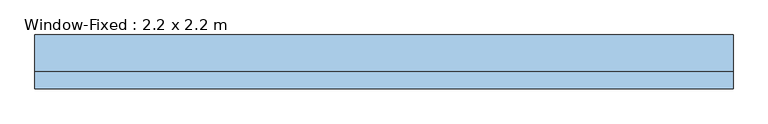
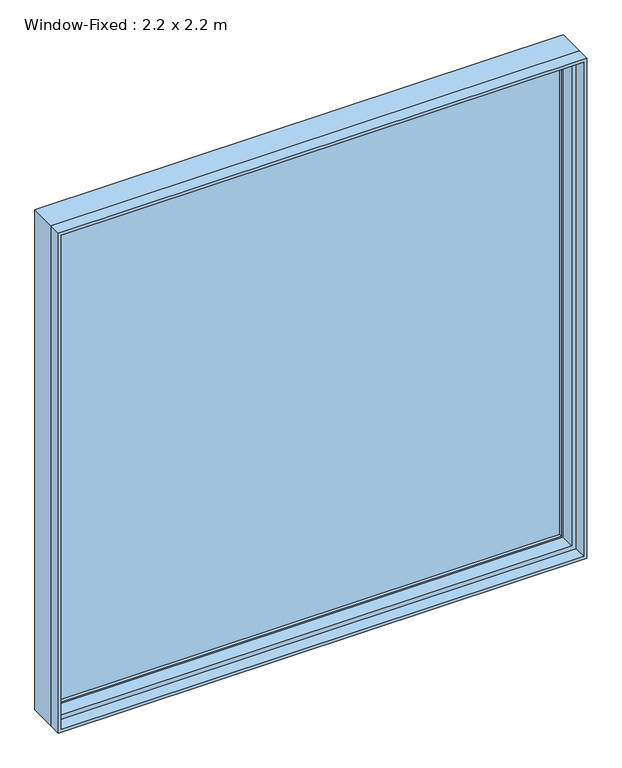
"""IFC4 building model written with IfcOpenShell, lengths in millimetres: window geometry, Window-Fixed : 2.2 x 2.2 m."""

from ifc_helpers import new_model, si_unit, frame, origin, place, context, project, spatial, polyline, outline, extrude, faceted_brep, source, transform, mapped, element, save


def window_fixed_2_2_x_2_2_m_8ae7ec15(model_context):
    return source(origin(), model_context, "Body", "SolidModel", [
        faceted_brep([(1100.0, -20.25, 3114.4), (1100.0, 94.05, 3114.4), (-1100.0, 94.05, 3114.4), (-1100.0, -20.25, 3114.4), (-1100.0, 94.05, 914.4), (-1100.0, -20.25, 914.4), (1100.0, 94.05, 914.4), (1100.0, -20.25, 914.4), (1068.25, -20.25, 3082.65), (1068.25, -20.25, 946.15), (-1068.25, -20.25, 946.15), (-1068.25, -20.25, 3082.65), (-1087.3, 94.05, 3101.7), (-1087.3, 94.05, 927.1), (1087.3, 94.05, 927.1), (1087.3, 94.05, 3101.7), (1068.25, 43.25, 3082.65), (-1068.25, 43.25, 3082.65), (1087.3, 43.25, 3101.7), (-1087.3, 43.25, 3101.7), (-1068.25, 43.25, 946.15), (-1087.3, 43.25, 927.1), (1068.25, 43.25, 946.15), (1087.3, 43.25, 927.1)], [[[0, 1, 2, 3]], [[3, 2, 4, 5]], [[5, 4, 6, 7]], [[3, 5, 7, 0], [8, 9, 10, 11]], [[7, 6, 1, 0]], [[1, 6, 4, 2], [12, 13, 14, 15]], [[16, 8, 11, 17]], [[15, 18, 19, 12]], [[17, 11, 10, 20]], [[12, 19, 21, 13]], [[20, 10, 9, 22]], [[13, 21, 23, 14]], [[22, 9, 8, 16]], [[18, 23, 21, 19], [17, 20, 22, 16]], [[14, 23, 18, 15]]]),
        extrude(outline(polyline([(3114.4, -1100.0), (914.4, -1100.0), (914.4, 1100.0), (3114.4, 1100.0), (3114.4, -1100.0)]), holes=[polyline([(3101.7, 1087.3), (927.1, 1087.3), (927.1, -1087.3), (3101.7, -1087.3), (3101.7, 1087.3)])]), frame((0.0, -75.0, 0.0), z_axis=(0.0, 1.0, 0.0), x_axis=(0.0, 0.0, 1.0)), (0.0, 0.0, 1.0), 54.75),
        extrude(outline(polyline([(927.1, 1087.3), (3101.7, 1087.3), (3101.7, -1087.3), (927.1, -1087.3), (927.1, 1087.3)]), holes=[polyline([(952.5, -1061.9), (3076.3, -1061.9), (3076.3, 1061.9), (952.5, 1061.9), (952.5, -1061.9)])]), frame((0.0, 43.25, 0.0), z_axis=(0.0, 1.0, 0.0), x_axis=(0.0, 0.0, 1.0)), (0.0, 0.0, 1.0), 44.45),
        extrude(outline(polyline([(1061.9, 75.0), (1061.9, 68.65), (-1061.9, 68.65), (-1061.9, 75.0), (1061.9, 75.0)])), frame((0.0, 0.0, 952.5), z_axis=(0.0, 0.0, 1.0), x_axis=(1.0, 0.0, 0.0)), (0.0, 0.0, 1.0), 2123.8),
        extrude(outline(polyline([(-1061.9, 55.95), (-1061.9, 62.3), (1061.9, 62.3), (1061.9, 55.95), (-1061.9, 55.95)])), frame((0.0, 0.0, 952.5), z_axis=(0.0, 0.0, 1.0), x_axis=(1.0, 0.0, 0.0)), (0.0, 0.0, 1.0), 2123.8),
    ])


if __name__ == "__main__":
    model = new_model("IFC4")
    model_context = context("Model", 3, world=origin())
    ifc_project = project(units=[si_unit("LENGTHUNIT", "METRE", prefix="MILLI")], contexts=[model_context])
    site = spatial("IfcSite", under=ifc_project)
    building = spatial("IfcBuilding", under=site)
    placement = place(None, origin())
    window_fixed_2_2_x_2_2_m_shape = window_fixed_2_2_x_2_2_m_8ae7ec15(model_context)
    element("IfcWindow", 1, ObjectType="Window-Fixed : 2.2 x 2.2 m", at=placement, inside=building, context=model_context, shape_type="MappedRepresentation", body=[
        mapped(window_fixed_2_2_x_2_2_m_shape, transform((0.0, 0.0, 0.0), x_axis=(1.0, 0.0, 0.0), y_axis=(0.0, 1.0, 0.0), z_axis=(0.0, 0.0, 1.0))),
    ])
    save(model, "model.ifc")

# Revit data of these elements
# Type "Window-Fixed : 2.2 x 2.2 m"
#   Type Mark = "44"
#   Fire Rating = "0.5h"
#   Analytic Construction = "Double glazing - domestic"
#   Window Inset [instance default] = 0 m
#   Wall Thickness [instance default] = 0.1524 m
#   Visual Light Transmittance = 0.81
#   Thermal Resistance (R) = 0.319569 (m²·K)/W
#   Solar Heat Gain Coefficient = 0.76
#   Rough Width = 2.2127 m
#   Rough Height = 2.2127 m
#   Interior Wall Closure [instance default] = 0.05715 m
#   Height = 2.2 m
#   Heat Transfer Coefficient (U) = 3.12929 W/(m²·K)
#   Frame Extension [instance default] = 0.00635 m
#   Exterior Wall Closure [instance default] = 0.03175 m
#   Extension Jamb [instance default] = 0.05715 m
#   Default Sill Height = 0.9144 m
#   Width = 2.2 m
#   Muntin Visibility = yes
#   Interior Trim Visibility [instance default] = yes
#   Exterior Trim Visibility [instance default] = yes
#   Extension Jamb Visibility [instance default] = yes
#   Muntin Pattern = Muntin Pattern_2x2 : Muntin Pattern_2x2
#   Interior Trim Material = Wood - Stained
#   Interior Trim = Trim-Window-Interior-Flat : Picture Frame
#   Interior Frame Material = Wood - Stained
#   Glass Panel Material = Glass
#   Exterior Trim Material = Clad - White
#   Exterior Trim = Trim-Window-Exterior-Flat : with Sill
#   Exterior Frame Material = Clad - White
#   Wall Closure = (empty or 0)
# Element 1 (IfcWindow, "Window-Fixed : 2.2 x 2.2 m")
#   Wall Thickness = 0.15 m
#   Extension Jamb = 0.05475 m
#   Materials on its faces: "Wood - Stained", "Glass", "Clad - White"
# Materials
#   "Wood - Stained": class "Wood", colour RGB 227 170 128, transparency 0, Cost = 0
#   "Glass": class "Glass", colour RGB 0 0 255, transparency 0.75, Description = "Soda Lime Glass", Cost = 0
#   "Clad - White": class "Wood", colour RGB 242 242 238, transparency 0, Cost = 0
